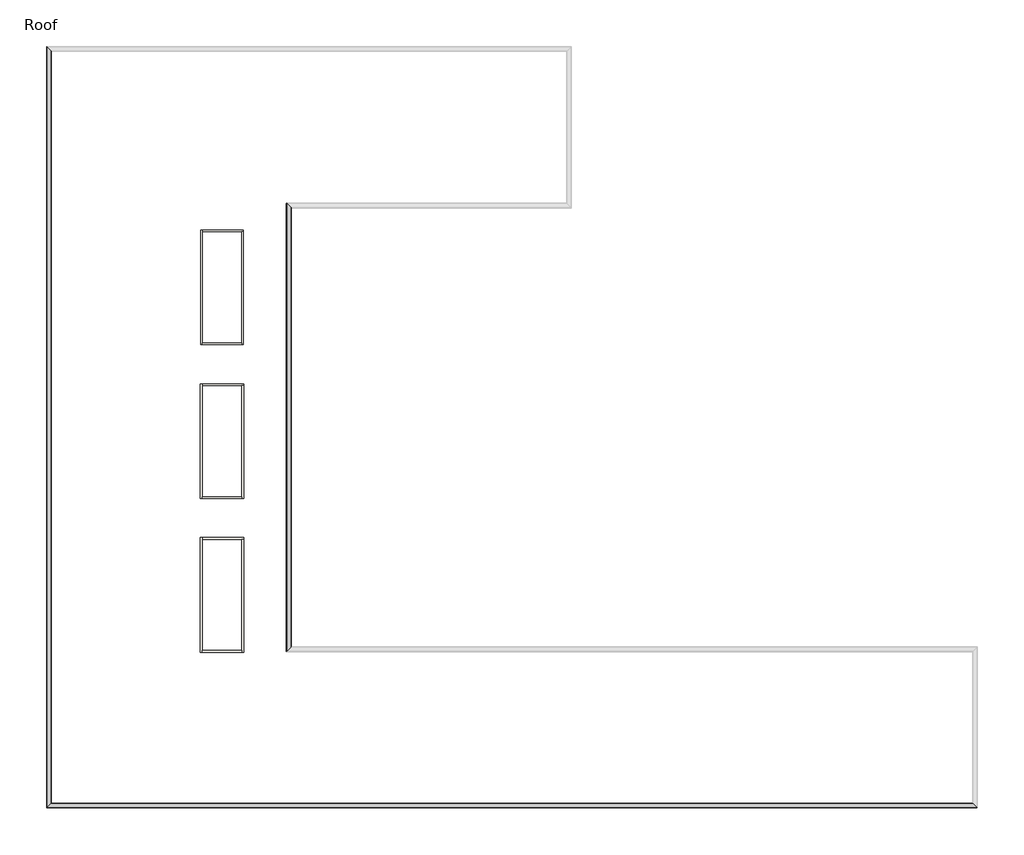
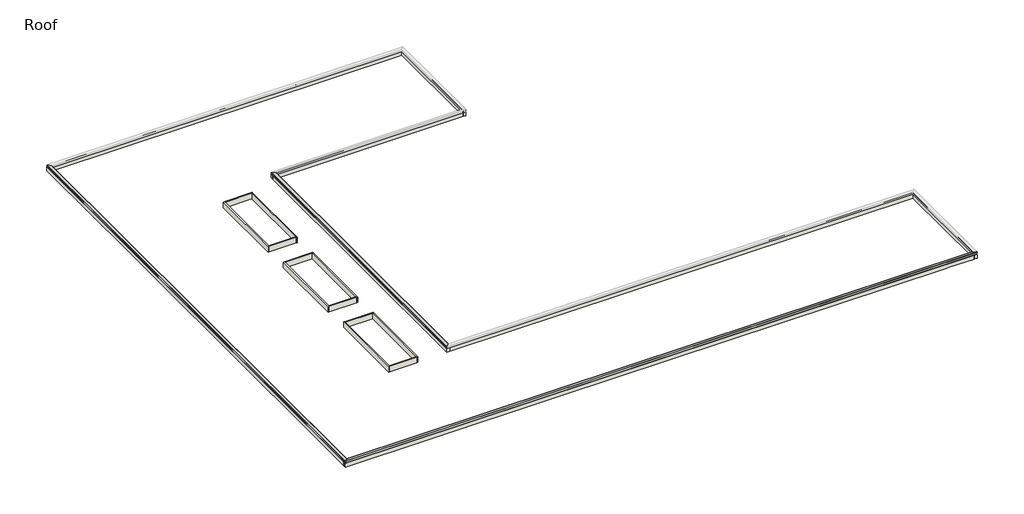
# One storey, part 1 of 2: 20 walls, 3 proxies.
"""IFC4 building model written with IfcOpenShell, lengths in millimetres."""

from ifc_helpers import new_model, si_unit, frame, origin, place, context, project, spatial, polyline, ellipse_curve, outline, extrude, faceted_brep, element, save
from ifc_brep_helpers import plane_surface, cylinder_surface, advanced_brep

model = new_model("IFC4")

# Units and contexts
model_context = context("Model", 3, world=origin())
ifc_project = project(units=[si_unit("LENGTHUNIT", "METRE", prefix="MILLI")], contexts=[model_context])

# Site, building, storey
site = spatial("IfcSite", under=ifc_project)
building = spatial("IfcBuilding", under=site)
storey = spatial("IfcBuildingStorey", under=building, Name="Roof", Elevation=10972.8)

# Proxies
placement = place(None, origin())
element("IfcBuildingElementProxy", 1, Name="Wall Sweeps", at=placement, inside=storey, context=model_context, shape_type="AdvancedBrep", body=[
    advanced_brep(
    [(17384.0457476, 42551.275, 11636.9329619), (17384.0457476, 42551.275, 11647.1824239), (17387.2207476, 42548.1, 11647.1824239), (17387.2207476, 42548.1, 11431.2824239), (17404.2349718, 42531.0857758, 11414.2681997), (17402.0062599, 42533.3144877, 11412.0394878), (17384.0457476, 42551.275, 11430.0), (17384.0457476, 42551.275, 11633.7462366), (17076.0707476, 42859.25, 11607.2537634), (17076.0707476, 42859.25, 11430.0), (17058.1102354, 42877.2105122, 11412.0394878), (17055.8651714, 42879.4555762, 11414.2845518), (17072.8957476, 42862.425, 11431.3151281), (17072.8957476, 42862.425, 11607.5268817), (17067.6672416, 42867.653506, 11607.0771178), (17068.7777162, 42866.5430314, 11609.8131313), (17384.0457476, 11201.325, 11636.9329619), (17068.7777162, 10886.0569685, 11609.8131313), (17067.6672416, 10884.9464939, 11607.0771178), (17072.8957476, 10890.175, 11607.5268817), (17072.8957476, 10890.175, 11431.3151281), (17055.8651714, 10873.1444237, 11414.2845518), (17058.1102354, 10875.3894877, 11412.0394878), (17076.0707476, 10893.35, 11430.0), (17076.0707476, 10893.35, 11607.2537634), (17384.0457476, 11201.325, 11633.7462366), (17384.0457476, 11201.325, 11430.0), (17402.0062599, 11219.2855122, 11412.0394878), (17404.2349718, 11221.5142242, 11414.2681997), (17387.2207476, 11204.5, 11431.2824239), (17387.2207476, 11204.5, 11647.1824239), (17384.0457476, 11201.325, 11647.1824239)],
    [
        (0, 1),
        (1, 2, ellipse_curve(frame((17385.6332476, 42549.6875, 11647.1824239), z_axis=(0.7071067811865511, 0.707106781186544, 0.0), x_axis=(-0.707106781186544, 0.707106781186551, 0.0)), 2.245064, 1.5875)),
        (2, 3),
        (3, 4),
        (4, 5),
        (5, 6),
        (6, 7),
        (7, 8),
        (8, 9),
        (9, 10),
        (10, 11),
        (11, 12),
        (12, 13),
        (13, 14),
        (14, 15, ellipse_curve(frame((17067.6672416, 42867.653506, 11608.6704804), z_axis=(0.7071067811865511, 0.707106781186544, 0.0), x_axis=(-0.707106781186544, 0.707106781186551, 0.0)), 2.2533551, 1.5933627)),
        (15, 0),
        (16, 17),
        (17, 18, ellipse_curve(frame((17067.6672416, 10884.9464939, 11608.6704804), z_axis=(0.7071067811865476, -0.7071067811865476, 0.0), x_axis=(0.7071067811865477, 0.7071067811865474, 0.0)), 2.2533551, 1.5933627)),
        (18, 19),
        (19, 20),
        (20, 21),
        (21, 22),
        (22, 23),
        (23, 24),
        (24, 25),
        (25, 26),
        (26, 27),
        (27, 28),
        (28, 29),
        (29, 30),
        (30, 31, ellipse_curve(frame((17385.6332476, 11202.9125, 11647.1824239), z_axis=(0.7071067811865476, -0.7071067811865476, 0.0), x_axis=(0.7071067811865477, 0.7071067811865474, 0.0)), 2.245064, 1.5875)),
        (31, 16),
        (0, 16),
        (31, 1),
        (30, 2),
        (29, 3),
        (28, 4),
        (27, 5),
        (26, 6),
        (25, 7),
        (24, 8),
        (23, 9),
        (22, 10),
        (21, 11),
        (20, 12),
        (19, 13),
        (18, 14),
        (17, 15),
    ],
    [
        plane_surface(frame((17377.6957476, 42557.625, 11277.6), z_axis=(0.7071067811865511, 0.707106781186544, 0.0), x_axis=(0.707106781186544, -0.7071067811865511, 0.0))),
        plane_surface(frame((17377.6957476, 11194.975, 11277.6), z_axis=(0.7071067811865476, -0.7071067811865476, 0.0), x_axis=(0.7071067811865476, 0.7071067811865476, 0.0))),
        plane_surface(frame((17384.0457476, 42551.275, 11636.9329619), z_axis=(-1.0, 0.0, 0.0), x_axis=(0.0, -1.0, 0.0))),
        cylinder_surface(frame((17385.6332476, 42557.625, 11647.1824239), z_axis=(0.0, 1.0, 0.0), x_axis=(-1.0, 0.0, 0.0)), 1.5875),
        plane_surface(frame((17387.2207476, 42548.1, 11647.1824239), z_axis=(1.0, 0.0, 0.0), x_axis=(0.0, -1.0, 0.0))),
        plane_surface(frame((17387.2207476, 42548.1, 11431.2824239), z_axis=(0.7071067811865493, 0.0, 0.7071067811865457), x_axis=(0.0, -1.0, 0.0))),
        plane_surface(frame((17404.2349718, 42531.0857758, 11414.2681997), z_axis=(0.7071067811865459, 0.0, -0.7071067811865492), x_axis=(0.0, -1.0, 0.0))),
        plane_surface(frame((17402.0062599, 42533.3144877, 11412.0394878), z_axis=(-0.7071067811865472, 0.0, -0.7071067811865478), x_axis=(0.0, -1.0, 0.0))),
        plane_surface(frame((17384.0457476, 42551.275, 11430.0), z_axis=(-1.0, 0.0, 0.0), x_axis=(0.0, -1.0, 0.0))),
        plane_surface(frame((17384.0457476, 42551.275, 11633.7462366), z_axis=(0.08570499422239307, 0.0, -0.9963205578353483), x_axis=(0.0, -1.0, 0.0))),
        plane_surface(frame((17076.0707476, 42859.25, 11607.2537634), z_axis=(1.0, 0.0, 0.0), x_axis=(0.0, -1.0, 0.0))),
        plane_surface(frame((17076.0707476, 42859.25, 11430.0), z_axis=(0.707106781186549, 0.0, -0.707106781186546), x_axis=(0.0, -1.0, 0.0))),
        plane_surface(frame((17058.1102354, 42877.2105122, 11412.0394878), z_axis=(-0.7071067811865422, 0.0, -0.7071067811865529), x_axis=(0.0, -1.0, 0.0))),
        plane_surface(frame((17055.8651714, 42879.4555762, 11414.2845518), z_axis=(-0.7071067811865496, 0.0, 0.7071067811865456), x_axis=(0.0, -1.0, 0.0))),
        plane_surface(frame((17072.8957476, 42862.425, 11431.3151281), z_axis=(-1.0, 0.0, 0.0), x_axis=(0.0, -1.0, 0.0))),
        plane_surface(frame((17072.8957476, 42862.425, 11607.5268817), z_axis=(0.08570499422239307, 0.0, -0.9963205578353483), x_axis=(0.0, -1.0, 0.0))),
        cylinder_surface(frame((17067.6672416, 42557.625, 11608.6704804), z_axis=(0.0, 1.0, 0.0), x_axis=(-1.0, 0.0, 0.0)), 1.5933627),
        plane_surface(frame((17068.7777162, 42866.5430314, 11609.8131313), z_axis=(-0.08570499422239307, 0.0, 0.9963205578353483), x_axis=(0.0, -1.0, 0.0))),
    ],
    [
        (0, [[1, 2, 3, 4, 5, 6, 7, 8, 9, 10, 11, 12, 13, 14, 15, 16]]),
        (1, [[17, 18, 19, 20, 21, 22, 23, 24, 25, 26, 27, 28, 29, 30, 31, 32]]),
        (2, [[-1, 33, -32, 34]]),
        (3, [[-2, -34, -31, 35]]),
        (4, [[-3, -35, -30, 36]]),
        (5, [[-4, -36, -29, 37]]),
        (6, [[-5, -37, -28, 38]]),
        (7, [[-6, -38, -27, 39]]),
        (8, [[-7, -39, -26, 40]]),
        (9, [[-8, -40, -25, 41]]),
        (10, [[-9, -41, -24, 42]]),
        (11, [[-10, -42, -23, 43]]),
        (12, [[-11, -43, -22, 44]]),
        (13, [[-12, -44, -21, 45]]),
        (14, [[-13, -45, -20, 46]]),
        (15, [[-14, -46, -19, 47]]),
        (16, [[-15, -47, -18, 48]]),
        (17, [[-16, -48, -17, -33]]),
    ],
),
])
element("IfcBuildingElementProxy", 2, Name="Wall Sweeps", at=placement, inside=storey, context=model_context, shape_type="AdvancedBrep", body=[
    advanced_brep(
    [(66317.1457476, -260.425, 11636.9329619), (66317.1457476, -260.425, 11647.1824239), (66320.3207476, -263.6, 11647.1824239), (66320.3207476, -263.6, 11431.2824239), (66337.3349718, -280.6142242, 11414.2681997), (66335.1062599, -278.3855123, 11412.0394878), (66317.1457476, -260.425, 11430.0), (66317.1457476, -260.425, 11633.7462366), (66009.1707476, 47.55, 11607.2537634), (66009.1707476, 47.55, 11430.0), (65991.2102354, 65.5105122, 11412.0394878), (65988.9651714, 67.7555762, 11414.2845518), (66005.9957476, 50.725, 11431.3151281), (66005.9957476, 50.725, 11607.5268817), (66000.7672416, 55.953506, 11607.0771178), (66001.8777162, 54.8430314, 11609.8131313), (-34.0042524, -260.425, 11636.9329619), (281.2637791, 54.8430314, 11609.8131313), (282.3742537, 55.953506, 11607.0771178), (277.1457476, 50.725, 11607.5268817), (277.1457476, 50.725, 11431.3151281), (294.1763239, 67.7555762, 11414.2845518), (291.9312599, 65.5105122, 11412.0394878), (273.9707476, 47.55, 11430.0), (273.9707476, 47.55, 11607.2537634), (-34.0042524, -260.425, 11633.7462366), (-34.0042524, -260.425, 11430.0), (-51.9647646, -278.3855123, 11412.0394878), (-54.1934766, -280.6142242, 11414.2681997), (-37.1792524, -263.6, 11431.2824239), (-37.1792524, -263.6, 11647.1824239), (-34.0042524, -260.425, 11647.1824239)],
    [
        (0, 1),
        (1, 2, ellipse_curve(frame((66318.7332476, -262.0125, 11647.1824239), z_axis=(0.7071067811865456, 0.7071067811865496, 0.0), x_axis=(0.7071067811865496, -0.7071067811865456, 0.0)), 2.245064, 1.5875)),
        (2, 3),
        (3, 4),
        (4, 5),
        (5, 6),
        (6, 7),
        (7, 8),
        (8, 9),
        (9, 10),
        (10, 11),
        (11, 12),
        (12, 13),
        (13, 14),
        (14, 15, ellipse_curve(frame((66000.7672416, 55.953506, 11608.6704804), z_axis=(0.7071067811865456, 0.7071067811865496, 0.0), x_axis=(0.7071067811865496, -0.7071067811865456, 0.0)), 2.2533551, 1.5933627)),
        (15, 0),
        (16, 17),
        (17, 18, ellipse_curve(frame((282.3742537, 55.953506, 11608.6704804), z_axis=(-0.7071067811865459, 0.7071067811865492, 0.0), x_axis=(0.707106781186549, 0.7071067811865459, 0.0)), 2.2533551, 1.5933627)),
        (18, 19),
        (19, 20),
        (20, 21),
        (21, 22),
        (22, 23),
        (23, 24),
        (24, 25),
        (25, 26),
        (26, 27),
        (27, 28),
        (28, 29),
        (29, 30),
        (30, 31, ellipse_curve(frame((-35.5917524, -262.0125, 11647.1824239), z_axis=(-0.7071067811865459, 0.7071067811865492, 0.0), x_axis=(0.707106781186549, 0.7071067811865459, 0.0)), 2.245064, 1.5875)),
        (31, 16),
        (0, 16),
        (31, 1),
        (30, 2),
        (29, 3),
        (28, 4),
        (27, 5),
        (26, 6),
        (25, 7),
        (24, 8),
        (23, 9),
        (22, 10),
        (21, 11),
        (20, 12),
        (19, 13),
        (18, 14),
        (17, 15),
    ],
    [
        plane_surface(frame((66310.7957476, -254.075, 11887.2), z_axis=(0.7071067811865456, 0.7071067811865496, 0.0), x_axis=(-0.7071067811865496, 0.7071067811865456, 0.0))),
        plane_surface(frame((-27.6542524, -254.075, 11887.2), z_axis=(-0.7071067811865459, 0.7071067811865492, 0.0), x_axis=(0.7071067811865492, 0.7071067811865459, 0.0))),
        plane_surface(frame((66317.1457476, -260.425, 11636.9329619), z_axis=(0.0, 1.0, 0.0), x_axis=(-1.0, 0.0, 0.0))),
        cylinder_surface(frame((66310.7957476, -262.0125, 11647.1824239), z_axis=(1.0, 0.0, 0.0), x_axis=(0.0, 1.0, 0.0)), 1.5875),
        plane_surface(frame((66320.3207476, -263.6, 11647.1824239), z_axis=(0.0, -1.0, 0.0), x_axis=(-1.0, 0.0, 0.0))),
        plane_surface(frame((66320.3207476, -263.6, 11431.2824239), z_axis=(0.0, -0.7071067811865493, 0.7071067811865457), x_axis=(-1.0, 0.0, 0.0))),
        plane_surface(frame((66337.3349718, -280.6142242, 11414.2681997), z_axis=(0.0, -0.7071067811865459, -0.7071067811865492), x_axis=(-1.0, 0.0, 0.0))),
        plane_surface(frame((66335.1062599, -278.3855123, 11412.0394878), z_axis=(0.0, 0.7071067811865472, -0.7071067811865478), x_axis=(-1.0, 0.0, 0.0))),
        plane_surface(frame((66317.1457476, -260.425, 11430.0), z_axis=(0.0, 1.0, 0.0), x_axis=(-1.0, 0.0, 0.0))),
        plane_surface(frame((66317.1457476, -260.425, 11633.7462366), z_axis=(0.0, -0.08570499422239307, -0.9963205578353483), x_axis=(-1.0, 0.0, 0.0))),
        plane_surface(frame((66009.1707476, 47.55, 11607.2537634), z_axis=(0.0, -1.0, 0.0), x_axis=(-1.0, 0.0, 0.0))),
        plane_surface(frame((66009.1707476, 47.55, 11430.0), z_axis=(0.0, -0.707106781186549, -0.707106781186546), x_axis=(-1.0, 0.0, 0.0))),
        plane_surface(frame((65991.2102354, 65.5105122, 11412.0394878), z_axis=(0.0, 0.7071067811865422, -0.7071067811865529), x_axis=(-1.0, 0.0, 0.0))),
        plane_surface(frame((65988.9651714, 67.7555762, 11414.2845518), z_axis=(0.0, 0.7071067811865496, 0.7071067811865456), x_axis=(-1.0, 0.0, 0.0))),
        plane_surface(frame((66005.9957476, 50.725, 11431.3151281), z_axis=(0.0, 1.0, 0.0), x_axis=(-1.0, 0.0, 0.0))),
        plane_surface(frame((66005.9957476, 50.725, 11607.5268817), z_axis=(0.0, -0.08570499422239307, -0.9963205578353483), x_axis=(-1.0, 0.0, 0.0))),
        cylinder_surface(frame((66310.7957476, 55.953506, 11608.6704804), z_axis=(1.0, 0.0, 0.0), x_axis=(0.0, 1.0, 0.0)), 1.5933627),
        plane_surface(frame((66001.8777162, 54.8430314, 11609.8131313), z_axis=(0.0, 0.08570499422239307, 0.9963205578353483), x_axis=(-1.0, 0.0, 0.0))),
    ],
    [
        (0, [[1, 2, 3, 4, 5, 6, 7, 8, 9, 10, 11, 12, 13, 14, 15, 16]]),
        (1, [[17, 18, 19, 20, 21, 22, 23, 24, 25, 26, 27, 28, 29, 30, 31, 32]]),
        (2, [[-1, 33, -32, 34]]),
        (3, [[-2, -34, -31, 35]]),
        (4, [[-3, -35, -30, 36]]),
        (5, [[-4, -36, -29, 37]]),
        (6, [[-5, -37, -28, 38]]),
        (7, [[-6, -38, -27, 39]]),
        (8, [[-7, -39, -26, 40]]),
        (9, [[-8, -40, -25, 41]]),
        (10, [[-9, -41, -24, 42]]),
        (11, [[-10, -42, -23, 43]]),
        (12, [[-11, -43, -22, 44]]),
        (13, [[-12, -44, -21, 45]]),
        (14, [[-13, -45, -20, 46]]),
        (15, [[-14, -46, -19, 47]]),
        (16, [[-15, -47, -18, 48]]),
        (17, [[-16, -48, -17, -33]]),
    ],
),
])
element("IfcBuildingElementProxy", 3, Name="Wall Sweeps", at=placement, inside=storey, context=model_context, shape_type="AdvancedBrep", body=[
    advanced_brep(
    [(-34.0042524, -260.425, 11636.9329619), (-34.0042524, -260.425, 11647.1824239), (-37.1792524, -263.6, 11647.1824239), (-37.1792524, -263.6, 11431.2824239), (-54.1934766, -280.6142242, 11414.2681997), (-51.9647646, -278.3855123, 11412.0394878), (-34.0042524, -260.425, 11430.0), (-34.0042524, -260.425, 11633.7462366), (273.9707476, 47.55, 11607.2537634), (273.9707476, 47.55, 11430.0), (291.9312599, 65.5105122, 11412.0394878), (294.1763239, 67.7555762, 11414.2845518), (277.1457476, 50.725, 11431.3151281), (277.1457476, 50.725, 11607.5268817), (282.3742537, 55.953506, 11607.0771178), (281.2637791, 54.8430314, 11609.8131313), (-34.0042524, 54038.425, 11636.9329619), (281.2637791, 53723.1569685, 11609.8131313), (282.3742537, 53722.0464939, 11607.0771178), (277.1457476, 53727.275, 11607.5268817), (277.1457476, 53727.275, 11431.3151281), (294.1763239, 53710.2444237, 11414.2845518), (291.9312599, 53712.4894877, 11412.0394878), (273.9707476, 53730.45, 11430.0), (273.9707476, 53730.45, 11607.2537634), (-34.0042524, 54038.425, 11633.7462366), (-34.0042524, 54038.425, 11430.0), (-51.9647646, 54056.3855122, 11412.0394878), (-54.1934766, 54058.6142242, 11414.2681997), (-37.1792524, 54041.6, 11431.2824239), (-37.1792524, 54041.6, 11647.1824239), (-34.0042524, 54038.425, 11647.1824239)],
    [
        (0, 1),
        (1, 2, ellipse_curve(frame((-35.5917524, -262.0125, 11647.1824239), z_axis=(0.7071067811865459, -0.7071067811865492, 0.0), x_axis=(-0.7071067811865492, -0.7071067811865457, 0.0)), 2.245064, 1.5875)),
        (2, 3),
        (3, 4),
        (4, 5),
        (5, 6),
        (6, 7),
        (7, 8),
        (8, 9),
        (9, 10),
        (10, 11),
        (11, 12),
        (12, 13),
        (13, 14),
        (14, 15, ellipse_curve(frame((282.3742537, 55.953506, 11608.6704804), z_axis=(0.7071067811865459, -0.7071067811865492, 0.0), x_axis=(-0.7071067811865492, -0.7071067811865457, 0.0)), 2.2533551, 1.5933627)),
        (15, 0),
        (16, 17),
        (17, 18, ellipse_curve(frame((282.3742537, 53722.0464939, 11608.6704804), z_axis=(0.7071067811865507, 0.7071067811865445, 0.0), x_axis=(0.7071067811865445, -0.7071067811865505, 0.0)), 2.2533551, 1.5933627)),
        (18, 19),
        (19, 20),
        (20, 21),
        (21, 22),
        (22, 23),
        (23, 24),
        (24, 25),
        (25, 26),
        (26, 27),
        (27, 28),
        (28, 29),
        (29, 30),
        (30, 31, ellipse_curve(frame((-35.5917524, 54040.0125, 11647.1824239), z_axis=(0.7071067811865507, 0.7071067811865445, 0.0), x_axis=(0.7071067811865445, -0.7071067811865505, 0.0)), 2.245064, 1.5875)),
        (31, 16),
        (0, 16),
        (31, 1),
        (30, 2),
        (29, 3),
        (28, 4),
        (27, 5),
        (26, 6),
        (25, 7),
        (24, 8),
        (23, 9),
        (22, 10),
        (21, 11),
        (20, 12),
        (19, 13),
        (18, 14),
        (17, 15),
    ],
    [
        plane_surface(frame((-27.6542524, -254.075, 11887.2), z_axis=(0.7071067811865459, -0.7071067811865492, 0.0), x_axis=(0.7071067811865492, 0.7071067811865459, 0.0))),
        plane_surface(frame((-27.6542524, 54032.075, 11887.2), z_axis=(0.7071067811865507, 0.7071067811865445, 0.0), x_axis=(0.7071067811865445, -0.7071067811865507, 0.0))),
        plane_surface(frame((-34.0042524, -260.425, 11636.9329619), z_axis=(1.0, 0.0, 0.0), x_axis=(0.0, 1.0, 0.0))),
        cylinder_surface(frame((-35.5917524, -254.075, 11647.1824239), z_axis=(0.0, -1.0, 0.0), x_axis=(1.0, 0.0, 0.0)), 1.5875),
        plane_surface(frame((-37.1792524, -263.6, 11647.1824239), z_axis=(-1.0, 0.0, 0.0), x_axis=(0.0, 1.0, 0.0))),
        plane_surface(frame((-37.1792524, -263.6, 11431.2824239), z_axis=(-0.7071067811865493, 0.0, 0.7071067811865457), x_axis=(0.0, 1.0, 0.0))),
        plane_surface(frame((-54.1934766, -280.6142242, 11414.2681997), z_axis=(-0.7071067811865459, 0.0, -0.7071067811865492), x_axis=(0.0, 1.0, 0.0))),
        plane_surface(frame((-51.9647646, -278.3855123, 11412.0394878), z_axis=(0.7071067811865472, 0.0, -0.7071067811865478), x_axis=(0.0, 1.0, 0.0))),
        plane_surface(frame((-34.0042524, -260.425, 11430.0), z_axis=(1.0, 0.0, 0.0), x_axis=(0.0, 1.0, 0.0))),
        plane_surface(frame((-34.0042524, -260.425, 11633.7462366), z_axis=(-0.08570499422239307, 0.0, -0.9963205578353483), x_axis=(0.0, 1.0, 0.0))),
        plane_surface(frame((273.9707476, 47.55, 11607.2537634), z_axis=(-1.0, 0.0, 0.0), x_axis=(0.0, 1.0, 0.0))),
        plane_surface(frame((273.9707476, 47.55, 11430.0), z_axis=(-0.707106781186549, 0.0, -0.707106781186546), x_axis=(0.0, 1.0, 0.0))),
        plane_surface(frame((291.9312599, 65.5105122, 11412.0394878), z_axis=(0.7071067811865422, 0.0, -0.7071067811865529), x_axis=(0.0, 1.0, 0.0))),
        plane_surface(frame((294.1763239, 67.7555762, 11414.2845518), z_axis=(0.7071067811865496, 0.0, 0.7071067811865456), x_axis=(0.0, 1.0, 0.0))),
        plane_surface(frame((277.1457476, 50.725, 11431.3151281), z_axis=(1.0, 0.0, 0.0), x_axis=(0.0, 1.0, 0.0))),
        plane_surface(frame((277.1457476, 50.725, 11607.5268817), z_axis=(-0.08570499422239307, 0.0, -0.9963205578353483), x_axis=(0.0, 1.0, 0.0))),
        cylinder_surface(frame((282.3742537, -254.075, 11608.6704804), z_axis=(0.0, -1.0, 0.0), x_axis=(1.0, 0.0, 0.0)), 1.5933627),
        plane_surface(frame((281.2637791, 54.8430314, 11609.8131313), z_axis=(0.08570499422239307, 0.0, 0.9963205578353483), x_axis=(0.0, 1.0, 0.0))),
    ],
    [
        (0, [[1, 2, 3, 4, 5, 6, 7, 8, 9, 10, 11, 12, 13, 14, 15, 16]]),
        (1, [[17, 18, 19, 20, 21, 22, 23, 24, 25, 26, 27, 28, 29, 30, 31, 32]]),
        (2, [[-1, 33, -32, 34]]),
        (3, [[-2, -34, -31, 35]]),
        (4, [[-3, -35, -30, 36]]),
        (5, [[-4, -36, -29, 37]]),
        (6, [[-5, -37, -28, 38]]),
        (7, [[-6, -38, -27, 39]]),
        (8, [[-7, -39, -26, 40]]),
        (9, [[-8, -40, -25, 41]]),
        (10, [[-9, -41, -24, 42]]),
        (11, [[-10, -42, -23, 43]]),
        (12, [[-11, -43, -22, 44]]),
        (13, [[-12, -44, -21, 45]]),
        (14, [[-13, -45, -20, 46]]),
        (15, [[-14, -46, -19, 47]]),
        (16, [[-15, -47, -18, 48]]),
        (17, [[-16, -48, -17, -33]]),
    ],
),
])

# Walls
element("IfcWall", 4, ObjectType="Exterior - Parapet EIFS on CMU", at=placement, inside=storey, context=model_context, shape_type="Brep", body=[
    faceted_brep([(37059.5207476, 54032.075, 10972.8), (37059.5207476, 53736.8, 10972.8), (37059.5207476, 42852.9, 10972.8), (37059.5207476, 42557.625, 10972.8), (37059.5207476, 42557.625, 11582.4), (37059.5207476, 42852.9, 11582.4), (37059.5207476, 53736.8, 11582.4), (37059.5207476, 54032.075, 11582.4), (37354.7957476, 54032.075, 10972.8), (37354.7957476, 54032.075, 11582.4), (37354.7957476, 42557.625, 11582.4), (37354.7957476, 42557.625, 10972.8), (37354.7957476, 45545.3, 10972.8)], [[[0, 1, 2, 3, 4, 5, 6, 7]], [[8, 9, 10, 11, 12]], [[3, 2, 1, 0, 8, 12, 11]], [[7, 6, 5, 4, 10, 9]], [[4, 3, 11, 10]], [[0, 7, 9, 8]]]),
])
element("IfcWall", 5, ObjectType="Exterior - Parapet EIFS on CMU", at=placement, inside=storey, context=model_context, shape_type="Brep", body=[
    faceted_brep([(37059.5207476, 42852.9, 10972.8), (17082.4207476, 42852.9, 10972.8), (17082.4207476, 42852.9, 11582.4), (37059.5207476, 42852.9, 11582.4), (37059.5207476, 42557.625, 10972.8), (37059.5207476, 42557.625, 11582.4), (17377.6957476, 42557.625, 11582.4), (17082.4207476, 42557.625, 11582.4), (17082.4207476, 42557.625, 10972.8), (17377.6957476, 42557.625, 10972.8)], [[[0, 1, 2, 3]], [[4, 5, 6, 7, 8, 9]], [[1, 0, 4, 9, 8]], [[3, 2, 7, 6, 5]], [[2, 1, 8, 7]], [[0, 3, 5, 4]]]),
])
element("IfcWall", 6, ObjectType="Exterior - Parapet EIFS on CMU", at=placement, inside=storey, context=model_context, shape_type="Brep", body=[
    faceted_brep([(17082.4207476, 42557.625, 10972.8), (17082.4207476, 10899.7, 10972.8), (17082.4207476, 10899.7, 11582.4), (17082.4207476, 42557.625, 11582.4), (17377.6957476, 42557.625, 10972.8), (17377.6957476, 42557.625, 11582.4), (17377.6957476, 11194.975, 11582.4), (17377.6957476, 10899.7, 11582.4), (17377.6957476, 10899.7, 10972.8), (17377.6957476, 11194.975, 10972.8)], [[[0, 1, 2, 3]], [[4, 5, 6, 7, 8, 9]], [[1, 0, 4, 9, 8]], [[3, 2, 7, 6, 5]], [[2, 1, 8, 7]], [[0, 3, 5, 4]]]),
])
element("IfcWall", 7, ObjectType="Exterior - Parapet EIFS on CMU", at=placement, inside=storey, context=model_context, shape_type="Brep", body=[
    faceted_brep([(17377.6957476, 10899.7, 10972.8), (66015.5207476, 10899.7, 10972.8), (66310.7957476, 10899.7, 10972.8), (66310.7957476, 10899.7, 11582.4), (66015.5207476, 10899.7, 11582.4), (17377.6957476, 10899.7, 11582.4), (17377.6957476, 11194.975, 10972.8), (17377.6957476, 11194.975, 11582.4), (66310.7957476, 11194.975, 11582.4), (66310.7957476, 11194.975, 10972.8)], [[[0, 1, 2, 3, 4, 5]], [[6, 7, 8, 9]], [[2, 1, 0, 6, 9]], [[5, 4, 3, 8, 7]], [[3, 2, 9, 8]], [[0, 5, 7, 6]]]),
])
element("IfcWall", 8, ObjectType="Exterior - Parapet EIFS on CMU", at=placement, inside=storey, context=model_context, shape_type="Brep", body=[
    faceted_brep([(66015.5207476, 10899.7, 10972.8), (66015.5207476, 41.2, 10972.8), (66015.5207476, -254.075, 10972.8), (66015.5207476, -254.075, 11582.4), (66015.5207476, 41.2, 11582.4), (66015.5207476, 10899.7, 11582.4), (66310.7957476, 10899.7, 10972.8), (66310.7957476, 10899.7, 11582.4), (66310.7957476, -254.075, 11582.4), (66310.7957476, -254.075, 10972.8), (66310.7957476, 53.9, 10972.8), (66310.7957476, 8334.3, 10972.8)], [[[0, 1, 2, 3, 4, 5]], [[6, 7, 8, 9, 10, 11]], [[2, 1, 0, 6, 11, 10, 9]], [[5, 4, 3, 8, 7]], [[3, 2, 9, 8]], [[0, 5, 7, 6]]]),
])
element("IfcWall", 9, ObjectType="Exterior - Parapet EIFS on CMU", at=placement, inside=storey, context=model_context, shape_type="Brep", body=[
    faceted_brep([(66015.5207476, 41.2, 10972.8), (267.6207476, 41.2, 10972.8), (-27.6542524, 41.2, 10972.8), (-27.6542524, 41.2, 11582.4), (267.6207476, 41.2, 11582.4), (66015.5207476, 41.2, 11582.4), (66015.5207476, -254.075, 10972.8), (66015.5207476, -254.075, 11582.4), (-27.6542524, -254.075, 11582.4), (-27.6542524, -254.075, 10972.8), (8357.5207476, -254.075, 10972.8), (22422.7707476, -254.075, 10972.8), (63137.3832476, -254.075, 10972.8), (63356.4582476, -254.075, 10972.8), (66002.8207476, -254.075, 10972.8)], [[[0, 1, 2, 3, 4, 5]], [[6, 7, 8, 9, 10, 11, 12, 13, 14]], [[2, 1, 0, 6, 14, 13, 12, 11, 10, 9]], [[5, 4, 3, 8, 7]], [[3, 2, 9, 8]], [[0, 5, 7, 6]]]),
])
element("IfcWall", 10, ObjectType="Exterior - Parapet EIFS on CMU", at=placement, inside=storey, context=model_context, shape_type="Brep", body=[
    faceted_brep([(267.6207476, 41.2, 10972.8), (267.6207476, 53736.8, 10972.8), (267.6207476, 54032.075, 10972.8), (267.6207476, 54032.075, 11582.4), (267.6207476, 53736.8, 11582.4), (267.6207476, 41.2, 11582.4), (-27.6542524, 54032.075, 10972.8), (-27.6542524, 45735.8, 10972.8), (-27.6542524, 40173.2, 10972.8), (-27.6542524, 40097.0, 10972.8), (-27.6542524, 28590.8, 10972.8), (-27.6542524, 28514.6, 10972.8), (-27.6542524, 25638.05, 10972.8), (-27.6542524, 41.2, 10972.8), (-27.6542524, 41.2, 11582.4), (-27.6542524, 54032.075, 11582.4)], [[[0, 1, 2, 3, 4, 5]], [[6, 7, 8, 9, 10, 11, 12, 13, 14, 15]], [[2, 1, 0, 13, 12, 11, 10, 9, 8, 7, 6]], [[5, 4, 3, 15, 14]], [[0, 5, 14, 13]], [[3, 2, 6, 15]]]),
])
element("IfcWall", 11, ObjectType="Exterior - Parapet EIFS on CMU", at=placement, inside=storey, context=model_context, shape_type="Brep", body=[
    faceted_brep([(267.6207476, 53736.8, 10972.8), (37059.5207476, 53736.8, 10972.8), (37059.5207476, 53736.8, 11582.4), (267.6207476, 53736.8, 11582.4), (267.6207476, 54032.075, 10972.8), (267.6207476, 54032.075, 11582.4), (37059.5207476, 54032.075, 11582.4), (37059.5207476, 54032.075, 10972.8), (34405.2207476, 54032.075, 10972.8), (16485.5207476, 54032.075, 10972.8)], [[[0, 1, 2, 3]], [[4, 5, 6, 7, 8, 9]], [[1, 0, 4, 9, 8, 7]], [[3, 2, 6, 5]], [[2, 1, 7, 6]], [[0, 3, 5, 4]]]),
])
element("IfcWall", 12, ObjectType="Typ. Partition Wall", at=placement, inside=storey, context=model_context, shape_type="Brep", body=[
    faceted_brep([(13998.9313551, 19015.0, 10972.8), (11039.0313551, 19015.0, 10972.8), (11039.0313551, 19015.0, 11582.4), (13998.9313551, 19015.0, 11582.4), (13998.9313551, 18900.7, 10972.8), (13998.9313551, 18900.7, 11582.4), (13884.6313551, 18900.7, 11582.4), (11039.0313551, 18900.7, 11582.4), (11039.0313551, 18900.7, 10972.8), (13884.6313551, 18900.7, 10972.8)], [[[0, 1, 2, 3]], [[4, 5, 6, 7, 8, 9]], [[1, 0, 4, 9, 8]], [[3, 2, 7, 6, 5]], [[0, 3, 5, 4]], [[2, 1, 8, 7]]]),
])
element("IfcWall", 13, ObjectType="Typ. Partition Wall", at=placement, inside=storey, context=model_context, shape_type="Brep", body=[
    faceted_brep([(13998.9313551, 10836.2, 10972.8), (13998.9313551, 18900.7, 10972.8), (13998.9313551, 18900.7, 11582.4), (13998.9313551, 10836.2, 11582.4), (13884.6313551, 10836.2, 10972.8), (13884.6313551, 10836.2, 11582.4), (13884.6313551, 10950.5, 11582.4), (13884.6313551, 18900.7, 11582.4), (13884.6313551, 18900.7, 10972.8), (13884.6313551, 10950.5, 10972.8)], [[[0, 1, 2, 3]], [[4, 5, 6, 7, 8, 9]], [[1, 0, 4, 9, 8]], [[3, 2, 7, 6, 5]], [[0, 3, 5, 4]], [[2, 1, 8, 7]]]),
])
element("IfcWall", 14, ObjectType="Typ. Partition Wall", at=placement, inside=storey, context=model_context, shape_type="SweptSolid", body=[
    extrude(outline(polyline([(13884.6313551, 10836.2), (11039.0313551, 10836.2), (11039.0313551, 10950.5), (13884.6313551, 10950.5), (13884.6313551, 10836.2)])), frame((0.0, 0.0, 10972.8), z_axis=(0.0, 0.0, 1.0), x_axis=(1.0, 0.0, 0.0)), (0.0, 0.0, 1.0), 609.6),
])
element("IfcWall", 15, ObjectType="Typ. Partition Wall", at=placement, inside=storey, context=model_context, shape_type="Brep", body=[
    faceted_brep([(10924.7313551, 19015.0, 10972.8), (10924.7313551, 10836.2, 10972.8), (10924.7313551, 10836.2, 11582.4), (10924.7313551, 19015.0, 11582.4), (11039.0313551, 19015.0, 10972.8), (11039.0313551, 19015.0, 11582.4), (11039.0313551, 18900.7, 11582.4), (11039.0313551, 10950.5, 11582.4), (11039.0313551, 10836.2, 11582.4), (11039.0313551, 10836.2, 10972.8), (11039.0313551, 10950.5, 10972.8), (11039.0313551, 18900.7, 10972.8)], [[[0, 1, 2, 3]], [[4, 5, 6, 7, 8, 9, 10, 11]], [[1, 0, 4, 11, 10, 9]], [[3, 2, 8, 7, 6, 5]], [[0, 3, 5, 4]], [[2, 1, 9, 8]]]),
])
element("IfcWall", 16, ObjectType="Typ. Partition Wall", at=placement, inside=storey, context=model_context, shape_type="Brep", body=[
    faceted_brep([(13998.9313552, 29987.8, 10972.8), (11039.0313551, 29987.8, 10972.8), (11039.0313551, 29987.8, 11582.4), (13998.9313552, 29987.8, 11582.4), (13998.9313552, 29873.5, 10972.8), (13998.9313552, 29873.5, 11582.4), (13884.6313552, 29873.5, 11582.4), (11039.0313551, 29873.5, 11582.4), (11039.0313551, 29873.5, 10972.8), (13884.6313552, 29873.5, 10972.8)], [[[0, 1, 2, 3]], [[4, 5, 6, 7, 8, 9]], [[1, 0, 4, 9, 8]], [[3, 2, 7, 6, 5]], [[0, 3, 5, 4]], [[2, 1, 8, 7]]]),
])
element("IfcWall", 17, ObjectType="Typ. Partition Wall", at=placement, inside=storey, context=model_context, shape_type="Brep", body=[
    faceted_brep([(13998.9313552, 21809.0, 10972.8), (13998.9313552, 29873.5, 10972.8), (13998.9313552, 29873.5, 11582.4), (13998.9313552, 21809.0, 11582.4), (13884.6313552, 21809.0, 10972.8), (13884.6313552, 21809.0, 11582.4), (13884.6313552, 21923.3, 11582.4), (13884.6313552, 29873.5, 11582.4), (13884.6313552, 29873.5, 10972.8), (13884.6313552, 21923.3, 10972.8)], [[[0, 1, 2, 3]], [[4, 5, 6, 7, 8, 9]], [[1, 0, 4, 9, 8]], [[3, 2, 7, 6, 5]], [[0, 3, 5, 4]], [[2, 1, 8, 7]]]),
])
element("IfcWall", 18, ObjectType="Typ. Partition Wall", at=placement, inside=storey, context=model_context, shape_type="SweptSolid", body=[
    extrude(outline(polyline([(13884.6313552, 21809.0), (11039.0313551, 21809.0), (11039.0313551, 21923.3), (13884.6313552, 21923.3), (13884.6313552, 21809.0)])), frame((0.0, 0.0, 10972.8), z_axis=(0.0, 0.0, 1.0), x_axis=(1.0, 0.0, 0.0)), (0.0, 0.0, 1.0), 609.6),
])
element("IfcWall", 19, ObjectType="Typ. Partition Wall", at=placement, inside=storey, context=model_context, shape_type="Brep", body=[
    faceted_brep([(10924.7313551, 29987.8, 10972.8), (10924.7313551, 21809.0, 10972.8), (10924.7313551, 21809.0, 11582.4), (10924.7313551, 29987.8, 11582.4), (11039.0313551, 29987.8, 10972.8), (11039.0313551, 29987.8, 11582.4), (11039.0313551, 29873.5, 11582.4), (11039.0313551, 21923.3, 11582.4), (11039.0313551, 21809.0, 11582.4), (11039.0313551, 21809.0, 10972.8), (11039.0313551, 21923.3, 10972.8), (11039.0313551, 29873.5, 10972.8)], [[[0, 1, 2, 3]], [[4, 5, 6, 7, 8, 9, 10, 11]], [[1, 0, 4, 11, 10, 9]], [[3, 2, 8, 7, 6, 5]], [[0, 3, 5, 4]], [[2, 1, 9, 8]]]),
])
element("IfcWall", 20, ObjectType="Typ. Partition Wall", at=placement, inside=storey, context=model_context, shape_type="Brep", body=[
    faceted_brep([(13988.9313552, 40960.6, 10972.8), (11059.2313551, 40960.6, 10972.8), (11059.2313551, 40960.6, 11582.4), (13988.9313552, 40960.6, 11582.4), (13988.9313552, 40846.3, 10972.8), (13988.9313552, 40846.3, 11582.4), (13874.6313552, 40846.3, 11582.4), (11059.2313551, 40846.3, 11582.4), (11059.2313551, 40846.3, 10972.8), (13874.6313552, 40846.3, 10972.8)], [[[0, 1, 2, 3]], [[4, 5, 6, 7, 8, 9]], [[1, 0, 4, 9, 8]], [[3, 2, 7, 6, 5]], [[0, 3, 5, 4]], [[2, 1, 8, 7]]]),
])
element("IfcWall", 21, ObjectType="Typ. Partition Wall", at=placement, inside=storey, context=model_context, shape_type="Brep", body=[
    faceted_brep([(13988.9313552, 32781.8, 10972.8), (13988.9313552, 40846.3, 10972.8), (13988.9313552, 40846.3, 11582.4), (13988.9313552, 32781.8, 11582.4), (13874.6313552, 32781.8, 10972.8), (13874.6313552, 32781.8, 11582.4), (13874.6313552, 32896.1, 11582.4), (13874.6313552, 40846.3, 11582.4), (13874.6313552, 40846.3, 10972.8), (13874.6313552, 32896.1, 10972.8)], [[[0, 1, 2, 3]], [[4, 5, 6, 7, 8, 9]], [[1, 0, 4, 9, 8]], [[3, 2, 7, 6, 5]], [[0, 3, 5, 4]], [[2, 1, 8, 7]]]),
])
element("IfcWall", 22, ObjectType="Typ. Partition Wall", at=placement, inside=storey, context=model_context, shape_type="SweptSolid", body=[
    extrude(outline(polyline([(13874.6313552, 32781.8), (11059.2313551, 32781.8), (11059.2313551, 32896.1), (13874.6313552, 32896.1), (13874.6313552, 32781.8)])), frame((0.0, 0.0, 10972.8), z_axis=(0.0, 0.0, 1.0), x_axis=(1.0, 0.0, 0.0)), (0.0, 0.0, 1.0), 609.6),
])
element("IfcWall", 23, ObjectType="Typ. Partition Wall", at=placement, inside=storey, context=model_context, shape_type="Brep", body=[
    faceted_brep([(10944.9313551, 40960.6, 10972.8), (10944.9313551, 32781.8, 10972.8), (10944.9313551, 32781.8, 11582.4), (10944.9313551, 40960.6, 11582.4), (11059.2313551, 40960.6, 10972.8), (11059.2313551, 40960.6, 11582.4), (11059.2313551, 40846.3, 11582.4), (11059.2313551, 32896.1, 11582.4), (11059.2313551, 32781.8, 11582.4), (11059.2313551, 32781.8, 10972.8), (11059.2313551, 32896.1, 10972.8), (11059.2313551, 40846.3, 10972.8)], [[[0, 1, 2, 3]], [[4, 5, 6, 7, 8, 9, 10, 11]], [[1, 0, 4, 11, 10, 9]], [[3, 2, 8, 7, 6, 5]], [[0, 3, 5, 4]], [[2, 1, 9, 8]]]),
])

save(model, "model.ifc")

# Revit data of these elements
# Type "Exterior - Parapet EIFS on CMU"
#   Assembly Code = "B2010100"
#   Width = 0' - 11 5/8"
#   Layers, outside or top first: 0' - 4" "EIFS - Exterior Insulation and Finish System" (function 4); 0' - 0" "Air Barrier - Air Infiltration Barrier" (function 100); 0' - 7 5/8" "Masonry - Concrete Masonry Units" (function 1)
# Type "Typ. Partition Wall"
#   Assembly Code = "B2010"
#   Type Mark = "A1"
#   Width = 0' - 4 1/2"
#   Layers, outside or top first: 0' - 0 1/2" "Gypsum Wall Board" (function 1); 0' - 3 1/2" "Metal - Stud Layer" (function 1); 0' - 0 1/2" "Gypsum Wall Board" (function 1)
# Elements 1, 2, 3 (IfcBuildingElementProxy)
#   Phase Created = New Construction
#   Materials on its faces: "Metal - Aluminum"
# Elements 4, 5, 6, 7, 8, 9, 10, 11 (IfcWall, "Exterior - Parapet EIFS on CMU")
#   Top Offset = 0' - 0"
#   Base Offset = 0' - 0"
#   wall height = 2' - 0"
#   Phase Created = New Construction
#   Base Constraint = Roof
#   Top Constraint = Parapet
#   Materials on its faces: "EIFS - Exterior Insulation and Finish System", "Masonry - Concrete Masonry Units"
# Elements 12, 13, 15, 16, 17, 19, 20, 21, 23 (IfcWall, "Typ. Partition Wall")
#   Top Offset = 0' - 0"
#   Base Offset = 0' - 0"
#   wall height = 2' - 0"
#   Phase Created = New Construction
#   Base Constraint = Roof
#   Top Constraint = Parapet
#   Materials on its faces: "Gypsum Wall Board", "Default Wall"
# Elements 14, 18, 22 (IfcWall, "Typ. Partition Wall")
#   Top Offset = 0' - 0"
#   Base Offset = 0' - 0"
#   wall height = 2' - 0"
#   Phase Created = New Construction
#   Base Constraint = Roof
#   Top Constraint = Parapet
#   Materials on its faces: "Default Wall", "Gypsum Wall Board"
# Materials
#   "EIFS - Exterior Insulation and Finish System": class "Stucco", colour RGB 242 242 242, transparency 0, Description = "Exterior finish"
#   "Air Barrier - Air Infiltration Barrier": class "Miscellaneous", colour RGB 127 127 127, transparency 0
#   "Masonry - Concrete Masonry Units": class "Concrete", colour RGB 190 197 182, transparency 0
#   "Gypsum Wall Board": class "Paint", colour RGB 153 153 153, transparency 0, Description = "Interior finish"
#   "Metal - Stud Layer": class "Metal", colour RGB 199 199 199, transparency 0
#   "Metal - Aluminum": class "Metal", colour RGB 140 140 140, transparency 0
#   "Default Wall": class "Miscellaneous", colour RGB 128 128 128, transparency 0
